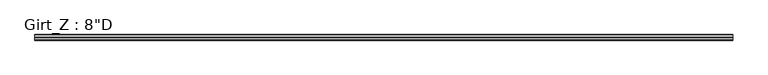
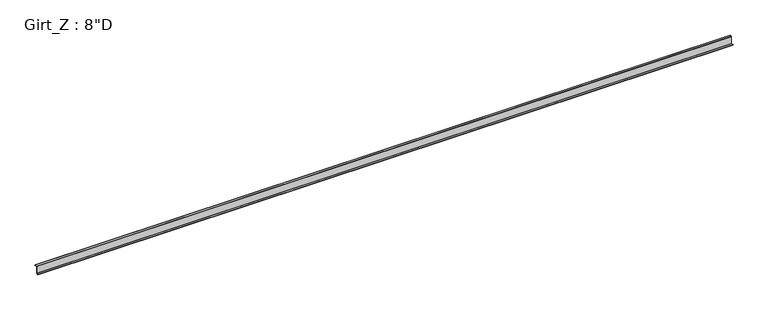
"""IFC4 building model written with IfcOpenShell, lengths in millimetres: beam geometry."""

from ifc_helpers import new_model, si_unit, point, frame, frame_2d, origin, place, context, project, spatial, polyline, circle_curve, trimmed, segment, composite_curve, outline, extrude, source, transform, mapped, element, save


def beam_935b8cdd(model_context):
    return source(origin(), model_context, "Body", "SweptSolid", [
        extrude(outline(composite_curve([segment(polyline([(63.5, 101.6), (75.745104, 87.0068534), (73.6169367, 85.221109), (62.204539, 98.821875), (3.3005807, 98.821875)]), True, "CONTINUOUS"), segment(trimmed(circle_curve(frame_2d((3.3741066, 96.8381931)), 1.9850441), [point((3.3005807, 98.821875))], [point((1.3890625, 96.8381931))], True, "CARTESIAN"), True, "CONTINUOUS"), segment(polyline([(1.3890625, 96.8381931), (1.3890625, -96.8375)]), True, "CONTINUOUS"), segment(trimmed(circle_curve(frame_2d((-3.3734375, -96.8375)), 4.7625), [point((1.3890625, -96.8375))], [point((-3.3734375, -101.6))], False, "CARTESIAN"), True, "CONTINUOUS"), segment(polyline([(-3.3734375, -101.6), (-63.5, -101.6), (-75.745104, -87.0068534), (-73.6169367, -85.221109), (-62.204539, -98.821875), (-3.2694106, -98.821875)]), True, "CONTINUOUS"), segment(trimmed(circle_curve(frame_2d((-3.3748024, -96.8389339)), 1.9857399), [point((-3.2694106, -98.821875))], [point((-1.3890625, -96.8389339))], True, "CARTESIAN"), True, "CONTINUOUS"), segment(polyline([(-1.3890625, -96.8389339), (-1.3890625, 96.8375)]), True, "CONTINUOUS"), segment(trimmed(circle_curve(frame_2d((3.3734375, 96.8375)), 4.7625), [point((-1.3890625, 96.8375))], [point((3.3734375, 101.6))], False, "CARTESIAN"), True, "CONTINUOUS"), segment(polyline([(3.3734375, 101.6), (63.5, 101.6)]), True, "CONTINUOUS")], self_intersect=False)), frame((-9323.6355469, 0.0, 0.0), z_axis=(1.0, 0.0, 0.0), x_axis=(0.0, 1.0, 0.0)), (0.0, 0.0, 1.0), 18647.2710937),
    ])


if __name__ == "__main__":
    model = new_model("IFC4")
    model_context = context("Model", 3, world=origin())
    ifc_project = project(units=[si_unit("LENGTHUNIT", "METRE", prefix="MILLI")], contexts=[model_context])
    site = spatial("IfcSite", under=ifc_project)
    building = spatial("IfcBuilding", under=site)
    placement = place(None, origin())
    beam_shape = beam_935b8cdd(model_context)
    element("IfcBeam", 1, ObjectType="Girt_Z : 8\"D", at=placement, inside=building, context=model_context, shape_type="MappedRepresentation", body=[
        mapped(beam_shape, transform((0.0, 0.0, 0.0), x_axis=(1.0, 0.0, 0.0), y_axis=(0.0, 1.0, 0.0), z_axis=(0.0, 0.0, 1.0))),
    ])
    save(model, "model.ifc")

# Revit data of these elements
# Type "Girt_Z : 8\"D"
#   Web_Thickness = 0' - 0 7/64"
#   Length [instance default] = 10' - 0"
#   Leg_1 = 0' - 2 1/2"
#   Height = 0' - 8"
#   Structural Material [instance default] = none
# Element 1 (IfcBeam, "Girt_Z : 8\"D")
#   Structural Material = Steel
#   Materials on its faces: "Steel"
# Materials
#   "Steel": class "Metal", colour RGB 118 118 114, transparency 0, Description = "Steel, mill finish", Cost = 0
